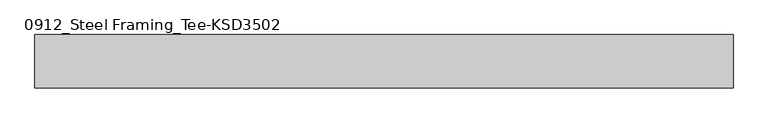
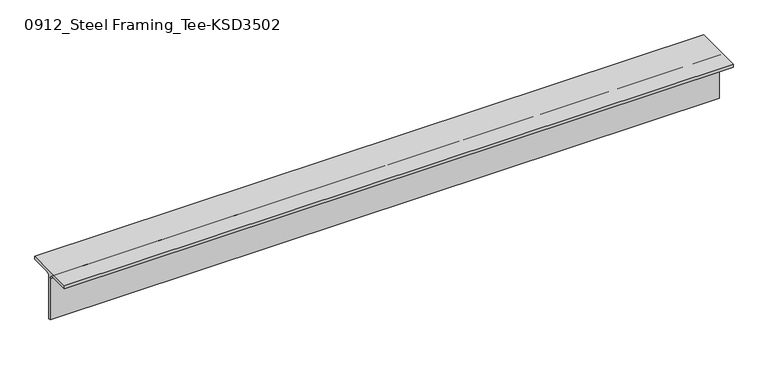
"""IFC4 building model written with IfcOpenShell, lengths in millimetres: member geometry, 0912_Steel Framing_Tee-KSD3502 : H_SB_ASB_CT-150x150x6.5x9."""

from ifc_helpers import new_model, si_unit, point, frame, frame_2d, origin, place, context, project, spatial, polyline, circle_curve, trimmed, segment, composite_curve, outline, extrude, source, transform, mapped, element, save


def member_0912_steel_framing_tee_ksd3502_353ddd1b(model_context):
    return source(origin(), model_context, "Body", "SweptSolid", [
        extrude(outline(composite_curve([segment(polyline([(-75.0, 75.0), (75.0, 75.0), (75.0, 66.0), (16.25, 66.0)]), True, "CONTINUOUS"), segment(trimmed(circle_curve(frame_2d((16.25, 53.0)), 13.0), [point((16.25, 66.0))], [point((3.25, 53.0))], True, "CARTESIAN"), True, "CONTINUOUS"), segment(polyline([(3.25, 53.0), (3.25, -75.0), (-3.25, -75.0), (-3.25, 53.0)]), True, "CONTINUOUS"), segment(trimmed(circle_curve(frame_2d((-16.25, 53.0)), 13.0), [point((-3.25, 53.0))], [point((-16.25, 66.0))], True, "CARTESIAN"), True, "CONTINUOUS"), segment(polyline([(-16.25, 66.0), (-75.0, 66.0), (-75.0, 75.0)]), True, "CONTINUOUS")], self_intersect=False)), frame((-1124.25, 0.0, 0.0), z_axis=(1.0, 0.0, 0.0), x_axis=(0.0, 1.0, 0.0)), (0.0, 0.0, 1.0), 1966.5),
    ])


if __name__ == "__main__":
    model = new_model("IFC4")
    model_context = context("Model", 3, world=origin())
    ifc_project = project(units=[si_unit("LENGTHUNIT", "METRE", prefix="MILLI")], contexts=[model_context])
    site = spatial("IfcSite", under=ifc_project)
    building = spatial("IfcBuilding", under=site)
    placement = place(None, origin())
    member_0912_steel_framing_tee_ksd3502_shape = member_0912_steel_framing_tee_ksd3502_353ddd1b(model_context)
    element("IfcMember", 1, ObjectType="0912_Steel Framing_Tee-KSD3502 : H_SB_ASB_CT-150x150x6.5x9", at=placement, inside=building, context=model_context, shape_type="MappedRepresentation", body=[
        mapped(member_0912_steel_framing_tee_ksd3502_shape, transform((0.0, 0.0, 0.0), x_axis=(1.0, 0.0, 0.0), y_axis=(0.0, 1.0, 0.0), z_axis=(0.0, 0.0, 1.0))),
    ])
    save(model, "model.ifc")

# Revit data of these elements
# Type "0912_Steel Framing_Tee-KSD3502 : H_SB_ASB_CT-150x150x6.5x9"
#   H_WM Code_1 = "S01AA003-00001 | Main Steel Structure Fabrication Work | Shelter/Building | Light Steel - Standard (30KG/M>Weight) | Material: (   )"
#   H_WM Code_2 = "S03AA029-00001 | Main Steel Structure Erection Work | Shelter/Building | Light Steel (30KG/M>Weight) | Material: (   )"
#   H_WM Code_3 = "S01AA010-00001 | Main Steel Structure Fabrication Work | Shelter/Building | Steel Painting/Coating | for Non-Fireproofed Steel Surface, Surface Preparation, Primer, Second & Final Coat | Material: (   )"
#   H_Q'ty Cal Type Tag = "SB-Q2"
#   Width = 15.0 cm
#   Web Thickness = 0.65 cm
#   Web Fillet = 1.3 cm
#   Section Area = 23.39 cm²
#   Perimeter = 0.60 m²/m
#   Nominal Weight = 18.40 kgf/m
#   Height = 15.0 cm
#   Flange Thickness = 0.9 cm
#   Centroid Vertical = 7.5 cm
#   Centroid Horizontal = 7.5 cm
#   Length [instance default] = 1.5000 m
#   Structural Material [instance default] = Steel, 45-345
#   Warping Constant = (empty or 0)
#   Torsional Moment of Inertia = 0
#   Section Name Key = ""
#   Plastic Modulus weak axis = 0
#   Plastic Modulus strong axis = 0
#   Moment of Inertia weak axis = 0
#   Moment of Inertia strong axis = 0
#   Elastic Modulus weak axis = 0
#   Elastic Modulus strong axis = 0
#   Bolt Spacing = 0
#   Assembly Code = ""
# Element 1 (IfcMember, "0912_Steel Framing_Tee-KSD3502 : H_SB_ASB_CT-150x150x6.5x9")
#   Structural Material = none
# Materials
#   "Steel, 45-345": class "Metal", colour RGB 189 187 185, transparency 0, Description = "Steel 345 MPa", Cost = 0
